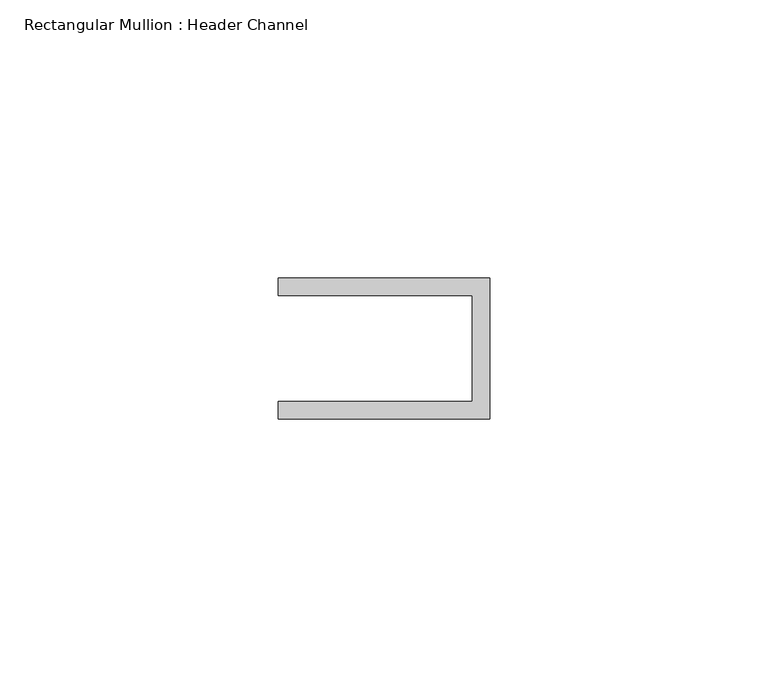
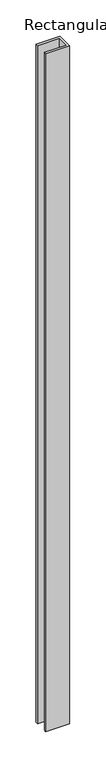
"""IFC4 building model written with IfcOpenShell, lengths in millimetres: member geometry, Rectangular Mullion : Header Channel."""

from ifc_helpers import new_model, si_unit, frame, origin, place, context, project, spatial, polyline, outline, extrude, source, transform, mapped, element, save


def rectangular_mullion_header_channel_079f7b39(model_context):
    return source(origin(), model_context, "Body", "SweptSolid", [
        extrude(outline(polyline([(0.0, 12.7), (0.0, -12.7), (-38.1, -12.7), (-38.1, -9.525), (-3.175, -9.525), (-3.175, 9.525), (-38.1, 9.525), (-38.1, 12.7), (0.0, 12.7)])), frame((0.0, 0.0, -1136.65), z_axis=(0.0, 0.0, 1.0), x_axis=(1.0, 0.0, 0.0)), (0.0, 0.0, 1.0), 1136.65),
    ])


if __name__ == "__main__":
    model = new_model("IFC4")
    model_context = context("Model", 3, world=origin())
    ifc_project = project(units=[si_unit("LENGTHUNIT", "METRE", prefix="MILLI")], contexts=[model_context])
    site = spatial("IfcSite", under=ifc_project)
    building = spatial("IfcBuilding", under=site)
    placement = place(None, origin())
    rectangular_mullion_header_channel_shape = rectangular_mullion_header_channel_079f7b39(model_context)
    element("IfcMember", 1, ObjectType="Rectangular Mullion : Header Channel", at=placement, inside=building, context=model_context, shape_type="MappedRepresentation", body=[
        mapped(rectangular_mullion_header_channel_shape, transform((0.0, 0.0, 0.0), x_axis=(1.0, 0.0, 0.0), y_axis=(0.0, 1.0, 0.0), z_axis=(0.0, 0.0, 1.0))),
    ])
    save(model, "model.ifc")

# Revit data of these elements
# Type "Rectangular Mullion : Header Channel"
#   built-in parameter 1007322 = 0.0833333 (stored number, unit not read)
#   built-in parameter 1007321 = -0.03125 (stored number, unit not read)
#   built-in parameter 1007320 = 0.0416667 (stored number, unit not read)
# Element 1 (IfcMember, "Rectangular Mullion : Header Channel")
#   Materials on its faces: "ALUM"
# Materials
#   "ALUM": class "Generic", colour RGB 157 157 157, transparency 0, Cost = 0
